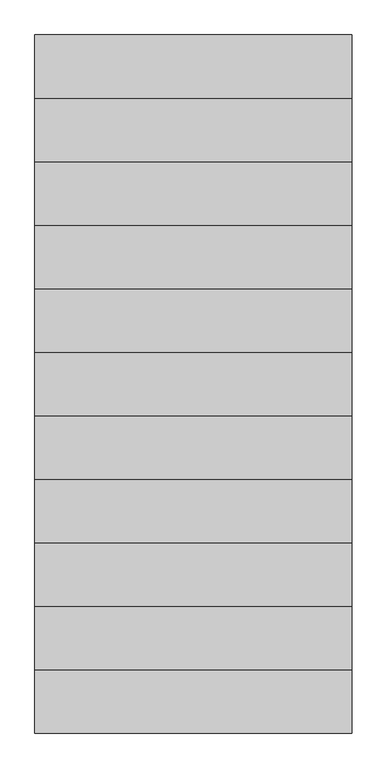
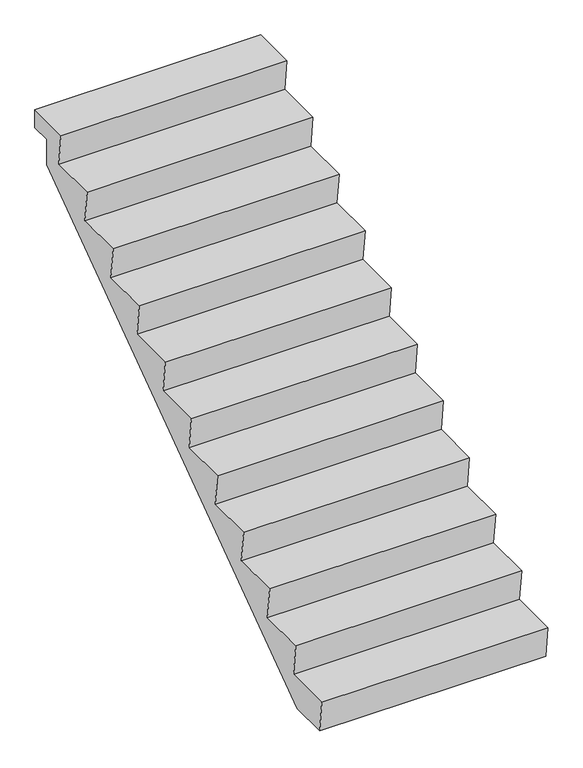
"""IFC4 building model written with IfcOpenShell, lengths in millimetres: stair geometry, NLRS_24_GM_LB_rechte steektrap prefab-AV_gen_rsf : prefab trap_gen__aant=11 b=1200 a=220 o=172.7 zonder bomen onder geen oplegnok."""

from ifc_helpers import new_model, si_unit, frame, origin, place, context, project, spatial, polyline, outline, extrude, source, transform, mapped, element, save


def stair_0bdb91d7(model_context):
    return source(origin(), model_context, "Body", "SweptSolid", [
        extrude(outline(polyline([(2400.0, 1900.0), (2640.0, 1900.0), (2640.0, 1800.0), (2530.0, 1800.0), (2530.0, 1658.5925892), (225.4292445, 0.0), (20.0, 0.0), (0.0, 172.7272727), (260.0, 172.7272727), (240.0, 345.4545455), (500.0, 345.4545455), (480.0, 518.1818182), (740.0, 518.1818182), (720.0, 690.9090909), (980.0, 690.9090909), (960.0, 863.6363636), (1220.0, 863.6363636), (1200.0, 1036.3636364), (1460.0, 1036.3636364), (1440.0, 1209.0909091), (1700.0, 1209.0909091), (1680.0, 1381.8181818), (1940.0, 1381.8181818), (1920.0, 1554.5454545), (2180.0, 1554.5454545), (2160.0, 1727.2727273), (2420.0, 1727.2727273), (2400.0, 1900.0)])), frame((-600.0, 0.0, 0.0), z_axis=(1.0, 0.0, 0.0), x_axis=(0.0, 1.0, 0.0)), (0.0, 0.0, 1.0), 1200.0),
    ])


if __name__ == "__main__":
    model = new_model("IFC4")
    model_context = context("Model", 3, world=origin())
    ifc_project = project(units=[si_unit("LENGTHUNIT", "METRE", prefix="MILLI")], contexts=[model_context])
    site = spatial("IfcSite", under=ifc_project)
    building = spatial("IfcBuilding", under=site)
    placement = place(None, origin())
    stair_shape = stair_0bdb91d7(model_context)
    element("IfcStair", 1, ObjectType="NLRS_24_GM_LB_rechte steektrap prefab-AV_gen_rsf : prefab trap_gen__aant=11 b=1200 a=220 o=172.7 zonder bomen onder geen oplegnok", at=placement, inside=building, context=model_context, shape_type="MappedRepresentation", body=[
        mapped(stair_shape, transform((0.0, 0.0, 0.0), x_axis=(1.0, 0.0, 0.0), y_axis=(0.0, 1.0, 0.0), z_axis=(0.0, 0.0, 1.0))),
    ])
    save(model, "model.ifc")

# Revit data of these elements
# Type "NLRS_24_GM_LB_rechte steektrap prefab-AV_gen_rsf : prefab trap_gen__aant=11 b=1200 a=220 o=172.7 zonder bomen onder geen oplegnok"
#   IfcExportAs = "IfcStair"
#   Type Comments = " "
#   Model = " "
#   Manufacturer = " "
#   Keynote = " "
#   Description = "rechte steektrap prefab\r\naant=11 b=1200 a=220 o=181,8\r\nzonder bomen"
#   Assembly Code = "24.11"
#   Aantrede onder = 240 mm
#   Width = 1200 mm
#   Wel diepte = 20 mm
#   Trapboom breedte = 0 mm
#   Thickness = 120 mm
#   Optrede onderste trede = 220 mm
#   NLRS_C_lengte = 2400 mm
#   Length = 2880 mm
#   Hoogte oplegnok onder = 100 mm
#   Hoogte oplegnok boven = 100 mm
#   Height = 1900 mm
#   Breedte oplegnok boven = 110 mm
#   BottomCalc = 220 mm
#   Actual Tread Depth = 240 mm
#   Actual Riser Height = 172.727 mm
#   Actual Number of Tread = 10
#   Actual Number of Risers = 11
#   Aantrede boven = 240 mm
#   Aantal treden max dertig = 11
#   Trapboom = no
#   Oplegnok onder = no
#   NLRS_C_materiaal = NLRS_f2_beton prefab_gen_rsf
#   Default Elevation = 0
# Element 1 (IfcStair, "NLRS_24_GM_LB_rechte steektrap prefab-AV_gen_rsf : prefab trap_gen__aant=11 b=1200 a=220 o=172.7 zonder bomen onder geen oplegnok")
#   Materials on its faces: "NLRS_f2_beton prefab_gen_rsf"
# Materials
#   "NLRS_f2_beton prefab_gen_rsf": class "F - Niet gebakken kunststeen", colour RGB 129 133 118, transparency 0, Keynote = "f2", Manufacturer = "Revit Standards Foundation", URL = "www.revitstandards.org", Description = "beton prefab", Cost = 0
